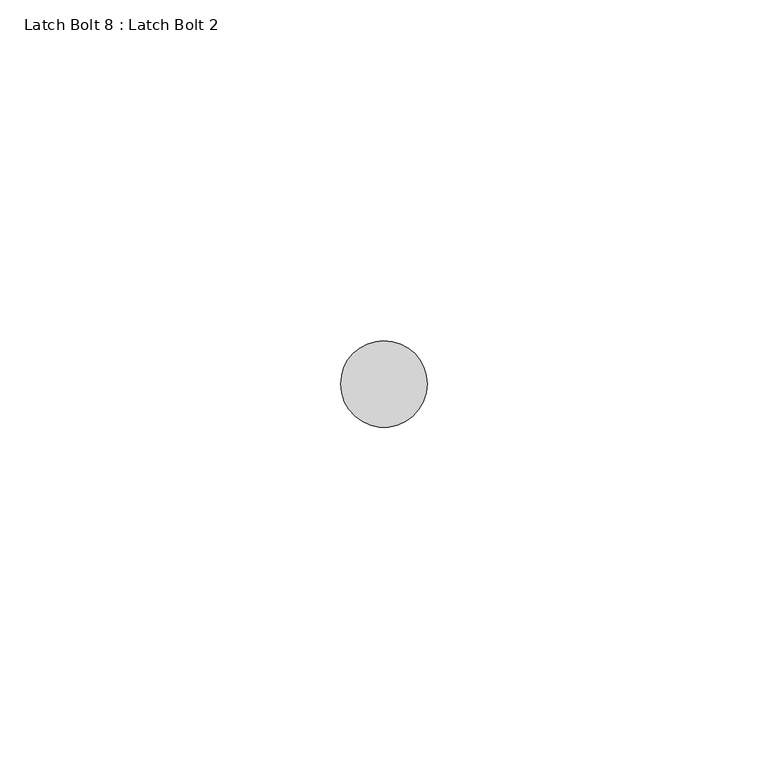
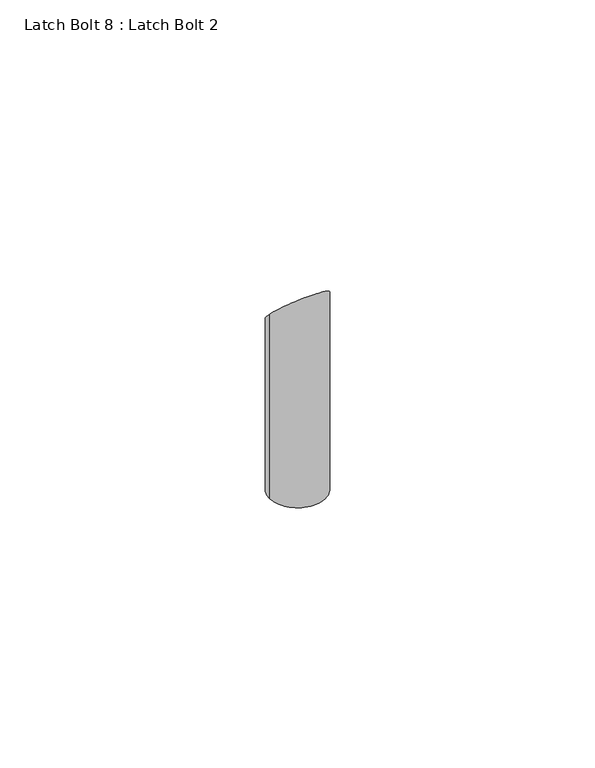
"""IFC4 building model written with IfcOpenShell, lengths in millimetres: proxy geometry, Latch Bolt 8 : Latch Bolt 2."""

from ifc_helpers import new_model, si_unit, frame, origin, place, context, project, spatial, circle_curve, ellipse_curve, source, transform, mapped, element, save
from ifc_brep_helpers import plane_surface, cylinder_surface, advanced_brep


def latch_bolt_8_latch_bolt_2_371a2b84(model_context):
    return source(origin(), model_context, "Body", "AdvancedBrep", [
        advanced_brep(
        [(587306.3384816, -532969.541467, 1022.35), (587319.0384816, -532969.541467, 1022.35), (587319.0384816, -532969.541467, 1066.7505507), (587306.3384816, -532969.541467, 1066.7505507), (587312.6884816, -532963.191467, 1060.4005507)],
        [
            (0, 1, circle_curve(frame((587312.6884816, -532969.541467, 1022.35), z_axis=(0.0, 0.0, -1.0), x_axis=(1.0, 0.0, 0.0)), 6.35)),
            (1, 0, circle_curve(frame((587312.6884816, -532969.541467, 1022.35), z_axis=(0.0, 0.0, -1.0), x_axis=(1.0, 0.0, 0.0)), 6.35)),
            (1, 2),
            (2, 3, ellipse_curve(frame((587312.6884816, -532969.541467, 1066.7505507), z_axis=(0.0, -0.7071067811861375, -0.7071067811869577), x_axis=(0.0, -0.7071067811869577, 0.7071067811861372)), 8.9802561, 6.35)),
            (3, 0),
            (3, 4, ellipse_curve(frame((587312.6884816, -532969.541467, 1066.7505507), z_axis=(0.0, -0.7071067811861375, -0.7071067811869577), x_axis=(0.0, -0.7071067811869577, 0.7071067811861372)), 8.9802561, 6.35)),
            (4, 2, ellipse_curve(frame((587312.6884816, -532969.541467, 1066.7505507), z_axis=(0.0, -0.7071067811861375, -0.7071067811869577), x_axis=(0.0, -0.7071067811869577, 0.7071067811861372)), 8.9802561, 6.35)),
        ],
        [
            plane_surface(frame((587319.0384816, -532969.541467, 1022.35), z_axis=(0.0, 0.0, -1.0), x_axis=(0.0, -1.0, 0.0))),
            cylinder_surface(frame((587312.6884816, -532969.541467, 1022.35), z_axis=(0.0, 0.0, 1.0), x_axis=(1.0, 0.0, 0.0)), 6.35),
            plane_surface(frame((587338.1185739, -532979.066467, 1076.2755507), z_axis=(0.0, 0.7071067811861375, 0.7071067811869577), x_axis=(-1.0, 0.0, 0.0))),
        ],
        [
            (0, [[1, 2]]),
            (1, [[-2, 3, 4, 5]]),
            (1, [[-1, -5, 6, 7, -3]]),
            (2, [[-4, -7, -6]]),
        ],
    ),
    ])


if __name__ == "__main__":
    model = new_model("IFC4")
    model_context = context("Model", 3, world=origin())
    ifc_project = project(units=[si_unit("LENGTHUNIT", "METRE", prefix="MILLI")], contexts=[model_context])
    site = spatial("IfcSite", under=ifc_project)
    building = spatial("IfcBuilding", under=site)
    placement = place(None, origin())
    latch_bolt_8_latch_bolt_2_shape = latch_bolt_8_latch_bolt_2_371a2b84(model_context)
    element("IfcBuildingElementProxy", 1, Name="Latch Bolt 8 : Latch Bolt 2", ObjectType="Latch Bolt 8 : Latch Bolt 2", at=placement, inside=building, context=model_context, shape_type="MappedRepresentation", body=[
        mapped(latch_bolt_8_latch_bolt_2_shape, transform((0.0, 0.0, 0.0), x_axis=(1.0, 0.0, 0.0), y_axis=(0.0, 1.0, 0.0), z_axis=(0.0, 0.0, 1.0))),
    ])
    save(model, "model.ifc")

# Revit data of these elements
# Element 1 (IfcBuildingElementProxy, "Latch Bolt 8 : Latch Bolt 2")
#   Materials on its faces: "GALV. GATE LATCH"
# Materials
#   "GALV. GATE LATCH": class "Metal", colour RGB 189 187 185, transparency 0, Description = "Carbon steel", Cost = 0
